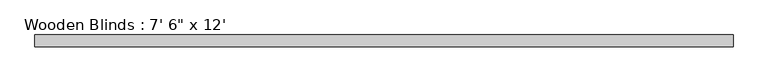
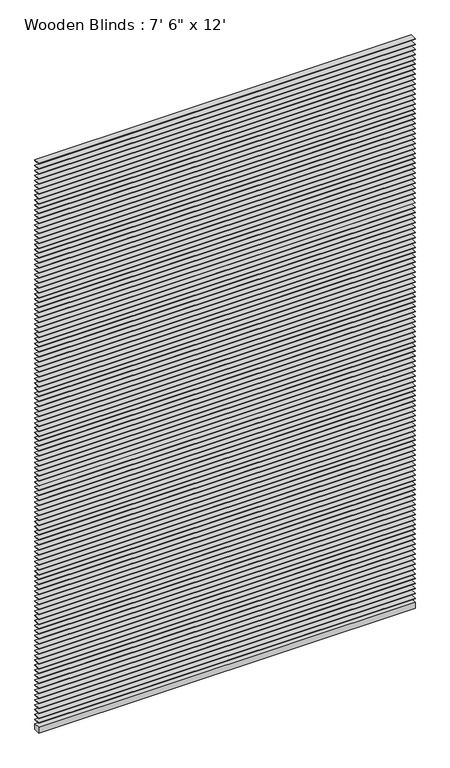
"""IFC4 building model written with IfcOpenShell, lengths in millimetres: furniture geometry."""

from ifc_helpers import new_model, si_unit, frame, origin, origin_with_axes, place, context, project, spatial, polyline, outline, extrude, source, transform, mapped, element, save


def furniture_480b9389(model_context):
    return source(origin(), model_context, "Body", "SweptSolid", [
        extrude(outline(polyline([(2286.0, 38.1), (2286.0, 0.0), (0.0, 0.0), (0.0, 38.1), (2286.0, 38.1)])), frame((0.0, 0.0, 3617.8790576), z_axis=(0.0, 0.0, 1.0), x_axis=(1.0, 0.0, 0.0)), (0.0, 0.0, 1.0), 3.175),
        extrude(outline(polyline([(2286.0, 38.1), (2286.0, 0.0), (0.0, 0.0), (0.0, 38.1), (2286.0, 38.1)])), frame((0.0, 0.0, 3586.1290576), z_axis=(0.0, 0.0, 1.0), x_axis=(1.0, 0.0, 0.0)), (0.0, 0.0, 1.0), 3.175),
        extrude(outline(polyline([(2286.0, 38.1), (2286.0, 0.0), (0.0, 0.0), (0.0, 38.1), (2286.0, 38.1)])), frame((0.0, 0.0, 3554.3790576), z_axis=(0.0, 0.0, 1.0), x_axis=(1.0, 0.0, 0.0)), (0.0, 0.0, 1.0), 3.175),
        extrude(outline(polyline([(2286.0, 38.1), (2286.0, 0.0), (0.0, 0.0), (0.0, 38.1), (2286.0, 38.1)])), frame((0.0, 0.0, 3522.6290576), z_axis=(0.0, 0.0, 1.0), x_axis=(1.0, 0.0, 0.0)), (0.0, 0.0, 1.0), 3.175),
        extrude(outline(polyline([(2286.0, 38.1), (2286.0, 0.0), (0.0, 0.0), (0.0, 38.1), (2286.0, 38.1)])), frame((0.0, 0.0, 3490.8790576), z_axis=(0.0, 0.0, 1.0), x_axis=(1.0, 0.0, 0.0)), (0.0, 0.0, 1.0), 3.175),
        extrude(outline(polyline([(2286.0, 38.1), (2286.0, 0.0), (0.0, 0.0), (0.0, 38.1), (2286.0, 38.1)])), frame((0.0, 0.0, 3459.1290576), z_axis=(0.0, 0.0, 1.0), x_axis=(1.0, 0.0, 0.0)), (0.0, 0.0, 1.0), 3.175),
        extrude(outline(polyline([(2286.0, 38.1), (2286.0, 0.0), (0.0, 0.0), (0.0, 38.1), (2286.0, 38.1)])), frame((0.0, 0.0, 3427.3790576), z_axis=(0.0, 0.0, 1.0), x_axis=(1.0, 0.0, 0.0)), (0.0, 0.0, 1.0), 3.175),
        extrude(outline(polyline([(2286.0, 38.1), (2286.0, 0.0), (0.0, 0.0), (0.0, 38.1), (2286.0, 38.1)])), frame((0.0, 0.0, 3395.6290576), z_axis=(0.0, 0.0, 1.0), x_axis=(1.0, 0.0, 0.0)), (0.0, 0.0, 1.0), 3.175),
        extrude(outline(polyline([(2286.0, 38.1), (2286.0, 0.0), (0.0, 0.0), (0.0, 38.1), (2286.0, 38.1)])), frame((0.0, 0.0, 3363.8790576), z_axis=(0.0, 0.0, 1.0), x_axis=(1.0, 0.0, 0.0)), (0.0, 0.0, 1.0), 3.175),
        extrude(outline(polyline([(2286.0, 38.1), (2286.0, 0.0), (0.0, 0.0), (0.0, 38.1), (2286.0, 38.1)])), frame((0.0, 0.0, 3332.1290576), z_axis=(0.0, 0.0, 1.0), x_axis=(1.0, 0.0, 0.0)), (0.0, 0.0, 1.0), 3.175),
        extrude(outline(polyline([(2286.0, 38.1), (2286.0, 0.0), (0.0, 0.0), (0.0, 38.1), (2286.0, 38.1)])), frame((0.0, 0.0, 3300.3790576), z_axis=(0.0, 0.0, 1.0), x_axis=(1.0, 0.0, 0.0)), (0.0, 0.0, 1.0), 3.175),
        extrude(outline(polyline([(2286.0, 38.1), (2286.0, 0.0), (0.0, 0.0), (0.0, 38.1), (2286.0, 38.1)])), frame((0.0, 0.0, 3268.6290576), z_axis=(0.0, 0.0, 1.0), x_axis=(1.0, 0.0, 0.0)), (0.0, 0.0, 1.0), 3.175),
        extrude(outline(polyline([(2286.0, 38.1), (2286.0, 0.0), (0.0, 0.0), (0.0, 38.1), (2286.0, 38.1)])), frame((0.0, 0.0, 3236.8790576), z_axis=(0.0, 0.0, 1.0), x_axis=(1.0, 0.0, 0.0)), (0.0, 0.0, 1.0), 3.175),
        extrude(outline(polyline([(2286.0, 38.1), (2286.0, 0.0), (0.0, 0.0), (0.0, 38.1), (2286.0, 38.1)])), frame((0.0, 0.0, 3205.1290576), z_axis=(0.0, 0.0, 1.0), x_axis=(1.0, 0.0, 0.0)), (0.0, 0.0, 1.0), 3.175),
        extrude(outline(polyline([(2286.0, 38.1), (2286.0, 0.0), (0.0, 0.0), (0.0, 38.1), (2286.0, 38.1)])), frame((0.0, 0.0, 3173.3790576), z_axis=(0.0, 0.0, 1.0), x_axis=(1.0, 0.0, 0.0)), (0.0, 0.0, 1.0), 3.175),
        extrude(outline(polyline([(2286.0, 38.1), (2286.0, 0.0), (0.0, 0.0), (0.0, 38.1), (2286.0, 38.1)])), frame((0.0, 0.0, 3141.6290576), z_axis=(0.0, 0.0, 1.0), x_axis=(1.0, 0.0, 0.0)), (0.0, 0.0, 1.0), 3.175),
        extrude(outline(polyline([(2286.0, 38.1), (2286.0, 0.0), (0.0, 0.0), (0.0, 38.1), (2286.0, 38.1)])), frame((0.0, 0.0, 3109.8790576), z_axis=(0.0, 0.0, 1.0), x_axis=(1.0, 0.0, 0.0)), (0.0, 0.0, 1.0), 3.175),
        extrude(outline(polyline([(2286.0, 38.1), (2286.0, 0.0), (0.0, 0.0), (0.0, 38.1), (2286.0, 38.1)])), frame((0.0, 0.0, 3078.1290576), z_axis=(0.0, 0.0, 1.0), x_axis=(1.0, 0.0, 0.0)), (0.0, 0.0, 1.0), 3.175),
        extrude(outline(polyline([(2286.0, 38.1), (2286.0, 0.0), (0.0, 0.0), (0.0, 38.1), (2286.0, 38.1)])), frame((0.0, 0.0, 3046.3790576), z_axis=(0.0, 0.0, 1.0), x_axis=(1.0, 0.0, 0.0)), (0.0, 0.0, 1.0), 3.175),
        extrude(outline(polyline([(2286.0, 38.1), (2286.0, 0.0), (0.0, 0.0), (0.0, 38.1), (2286.0, 38.1)])), frame((0.0, 0.0, 3014.6290576), z_axis=(0.0, 0.0, 1.0), x_axis=(1.0, 0.0, 0.0)), (0.0, 0.0, 1.0), 3.175),
        extrude(outline(polyline([(2286.0, 38.1), (2286.0, 0.0), (0.0, 0.0), (0.0, 38.1), (2286.0, 38.1)])), frame((0.0, 0.0, 2982.8790576), z_axis=(0.0, 0.0, 1.0), x_axis=(1.0, 0.0, 0.0)), (0.0, 0.0, 1.0), 3.175),
        extrude(outline(polyline([(2286.0, 38.1), (2286.0, 0.0), (0.0, 0.0), (0.0, 38.1), (2286.0, 38.1)])), frame((0.0, 0.0, 2951.1290576), z_axis=(0.0, 0.0, 1.0), x_axis=(1.0, 0.0, 0.0)), (0.0, 0.0, 1.0), 3.175),
        extrude(outline(polyline([(2286.0, 38.1), (2286.0, 0.0), (0.0, 0.0), (0.0, 38.1), (2286.0, 38.1)])), frame((0.0, 0.0, 2919.3790576), z_axis=(0.0, 0.0, 1.0), x_axis=(1.0, 0.0, 0.0)), (0.0, 0.0, 1.0), 3.175),
        extrude(outline(polyline([(2286.0, 38.1), (2286.0, 0.0), (0.0, 0.0), (0.0, 38.1), (2286.0, 38.1)])), frame((0.0, 0.0, 2887.6290576), z_axis=(0.0, 0.0, 1.0), x_axis=(1.0, 0.0, 0.0)), (0.0, 0.0, 1.0), 3.175),
        extrude(outline(polyline([(2286.0, 38.1), (2286.0, 0.0), (0.0, 0.0), (0.0, 38.1), (2286.0, 38.1)])), frame((0.0, 0.0, 2855.8790576), z_axis=(0.0, 0.0, 1.0), x_axis=(1.0, 0.0, 0.0)), (0.0, 0.0, 1.0), 3.175),
        extrude(outline(polyline([(2286.0, 38.1), (2286.0, 0.0), (0.0, 0.0), (0.0, 38.1), (2286.0, 38.1)])), frame((0.0, 0.0, 2824.1290576), z_axis=(0.0, 0.0, 1.0), x_axis=(1.0, 0.0, 0.0)), (0.0, 0.0, 1.0), 3.175),
        extrude(outline(polyline([(2286.0, 38.1), (2286.0, 0.0), (0.0, 0.0), (0.0, 38.1), (2286.0, 38.1)])), frame((0.0, 0.0, 2792.3790576), z_axis=(0.0, 0.0, 1.0), x_axis=(1.0, 0.0, 0.0)), (0.0, 0.0, 1.0), 3.175),
        extrude(outline(polyline([(2286.0, 38.1), (2286.0, 0.0), (0.0, 0.0), (0.0, 38.1), (2286.0, 38.1)])), frame((0.0, 0.0, 2760.6290576), z_axis=(0.0, 0.0, 1.0), x_axis=(1.0, 0.0, 0.0)), (0.0, 0.0, 1.0), 3.175),
        extrude(outline(polyline([(2286.0, 38.1), (2286.0, 0.0), (0.0, 0.0), (0.0, 38.1), (2286.0, 38.1)])), frame((0.0, 0.0, 2728.8790576), z_axis=(0.0, 0.0, 1.0), x_axis=(1.0, 0.0, 0.0)), (0.0, 0.0, 1.0), 3.175),
        extrude(outline(polyline([(2286.0, 38.1), (2286.0, 0.0), (0.0, 0.0), (0.0, 38.1), (2286.0, 38.1)])), frame((0.0, 0.0, 2697.1290576), z_axis=(0.0, 0.0, 1.0), x_axis=(1.0, 0.0, 0.0)), (0.0, 0.0, 1.0), 3.175),
        extrude(outline(polyline([(2286.0, 38.1), (2286.0, 0.0), (0.0, 0.0), (0.0, 38.1), (2286.0, 38.1)])), frame((0.0, 0.0, 2665.3790576), z_axis=(0.0, 0.0, 1.0), x_axis=(1.0, 0.0, 0.0)), (0.0, 0.0, 1.0), 3.175),
        extrude(outline(polyline([(2286.0, 38.1), (2286.0, 0.0), (0.0, 0.0), (0.0, 38.1), (2286.0, 38.1)])), frame((0.0, 0.0, 2633.6290576), z_axis=(0.0, 0.0, 1.0), x_axis=(1.0, 0.0, 0.0)), (0.0, 0.0, 1.0), 3.175),
        extrude(outline(polyline([(2286.0, 38.1), (2286.0, 0.0), (0.0, 0.0), (0.0, 38.1), (2286.0, 38.1)])), frame((0.0, 0.0, 2601.8790576), z_axis=(0.0, 0.0, 1.0), x_axis=(1.0, 0.0, 0.0)), (0.0, 0.0, 1.0), 3.175),
        extrude(outline(polyline([(2286.0, 38.1), (2286.0, 0.0), (0.0, 0.0), (0.0, 38.1), (2286.0, 38.1)])), frame((0.0, 0.0, 2570.1290576), z_axis=(0.0, 0.0, 1.0), x_axis=(1.0, 0.0, 0.0)), (0.0, 0.0, 1.0), 3.175),
        extrude(outline(polyline([(2286.0, 38.1), (2286.0, 0.0), (0.0, 0.0), (0.0, 38.1), (2286.0, 38.1)])), frame((0.0, 0.0, 2538.3790576), z_axis=(0.0, 0.0, 1.0), x_axis=(1.0, 0.0, 0.0)), (0.0, 0.0, 1.0), 3.175),
        extrude(outline(polyline([(2286.0, 38.1), (2286.0, 0.0), (0.0, 0.0), (0.0, 38.1), (2286.0, 38.1)])), frame((0.0, 0.0, 2506.6290576), z_axis=(0.0, 0.0, 1.0), x_axis=(1.0, 0.0, 0.0)), (0.0, 0.0, 1.0), 3.175),
        extrude(outline(polyline([(2286.0, 38.1), (2286.0, 0.0), (0.0, 0.0), (0.0, 38.1), (2286.0, 38.1)])), frame((0.0, 0.0, 2474.8790576), z_axis=(0.0, 0.0, 1.0), x_axis=(1.0, 0.0, 0.0)), (0.0, 0.0, 1.0), 3.175),
        extrude(outline(polyline([(2286.0, 38.1), (2286.0, 0.0), (0.0, 0.0), (0.0, 38.1), (2286.0, 38.1)])), frame((0.0, 0.0, 2443.1290576), z_axis=(0.0, 0.0, 1.0), x_axis=(1.0, 0.0, 0.0)), (0.0, 0.0, 1.0), 3.175),
        extrude(outline(polyline([(2286.0, 38.1), (2286.0, 0.0), (0.0, 0.0), (0.0, 38.1), (2286.0, 38.1)])), frame((0.0, 0.0, 2411.3790576), z_axis=(0.0, 0.0, 1.0), x_axis=(1.0, 0.0, 0.0)), (0.0, 0.0, 1.0), 3.175),
        extrude(outline(polyline([(2286.0, 38.1), (2286.0, 0.0), (0.0, 0.0), (0.0, 38.1), (2286.0, 38.1)])), frame((0.0, 0.0, 2379.6290576), z_axis=(0.0, 0.0, 1.0), x_axis=(1.0, 0.0, 0.0)), (0.0, 0.0, 1.0), 3.175),
        extrude(outline(polyline([(2286.0, 38.1), (2286.0, 0.0), (0.0, 0.0), (0.0, 38.1), (2286.0, 38.1)])), frame((0.0, 0.0, 2347.8790576), z_axis=(0.0, 0.0, 1.0), x_axis=(1.0, 0.0, 0.0)), (0.0, 0.0, 1.0), 3.175),
        extrude(outline(polyline([(2286.0, 38.1), (2286.0, 0.0), (0.0, 0.0), (0.0, 38.1), (2286.0, 38.1)])), frame((0.0, 0.0, 2316.1290576), z_axis=(0.0, 0.0, 1.0), x_axis=(1.0, 0.0, 0.0)), (0.0, 0.0, 1.0), 3.175),
        extrude(outline(polyline([(2286.0, 38.1), (2286.0, 0.0), (0.0, 0.0), (0.0, 38.1), (2286.0, 38.1)])), frame((0.0, 0.0, 2284.3790576), z_axis=(0.0, 0.0, 1.0), x_axis=(1.0, 0.0, 0.0)), (0.0, 0.0, 1.0), 3.175),
        extrude(outline(polyline([(2286.0, 38.1), (2286.0, 0.0), (0.0, 0.0), (0.0, 38.1), (2286.0, 38.1)])), frame((0.0, 0.0, 2252.6290576), z_axis=(0.0, 0.0, 1.0), x_axis=(1.0, 0.0, 0.0)), (0.0, 0.0, 1.0), 3.175),
        extrude(outline(polyline([(2286.0, 38.1), (2286.0, 0.0), (0.0, 0.0), (0.0, 38.1), (2286.0, 38.1)])), frame((0.0, 0.0, 2220.8790576), z_axis=(0.0, 0.0, 1.0), x_axis=(1.0, 0.0, 0.0)), (0.0, 0.0, 1.0), 3.175),
        extrude(outline(polyline([(2286.0, 38.1), (2286.0, 0.0), (0.0, 0.0), (0.0, 38.1), (2286.0, 38.1)])), frame((0.0, 0.0, 2189.1290576), z_axis=(0.0, 0.0, 1.0), x_axis=(1.0, 0.0, 0.0)), (0.0, 0.0, 1.0), 3.175),
        extrude(outline(polyline([(2286.0, 38.1), (2286.0, 0.0), (0.0, 0.0), (0.0, 38.1), (2286.0, 38.1)])), frame((0.0, 0.0, 2157.3790576), z_axis=(0.0, 0.0, 1.0), x_axis=(1.0, 0.0, 0.0)), (0.0, 0.0, 1.0), 3.175),
        extrude(outline(polyline([(2286.0, 38.1), (2286.0, 0.0), (0.0, 0.0), (0.0, 38.1), (2286.0, 38.1)])), frame((0.0, 0.0, 2125.6290576), z_axis=(0.0, 0.0, 1.0), x_axis=(1.0, 0.0, 0.0)), (0.0, 0.0, 1.0), 3.175),
        extrude(outline(polyline([(2286.0, 38.1), (2286.0, 0.0), (0.0, 0.0), (0.0, 38.1), (2286.0, 38.1)])), frame((0.0, 0.0, 2093.8790576), z_axis=(0.0, 0.0, 1.0), x_axis=(1.0, 0.0, 0.0)), (0.0, 0.0, 1.0), 3.175),
        extrude(outline(polyline([(2286.0, 38.1), (2286.0, 0.0), (0.0, 0.0), (0.0, 38.1), (2286.0, 38.1)])), frame((0.0, 0.0, 2062.1290576), z_axis=(0.0, 0.0, 1.0), x_axis=(1.0, 0.0, 0.0)), (0.0, 0.0, 1.0), 3.175),
        extrude(outline(polyline([(2286.0, 38.1), (2286.0, 0.0), (0.0, 0.0), (0.0, 38.1), (2286.0, 38.1)])), frame((0.0, 0.0, 2030.3790576), z_axis=(0.0, 0.0, 1.0), x_axis=(1.0, 0.0, 0.0)), (0.0, 0.0, 1.0), 3.175),
        extrude(outline(polyline([(2286.0, 38.1), (2286.0, 0.0), (0.0, 0.0), (0.0, 38.1), (2286.0, 38.1)])), frame((0.0, 0.0, 1998.6290576), z_axis=(0.0, 0.0, 1.0), x_axis=(1.0, 0.0, 0.0)), (0.0, 0.0, 1.0), 3.175),
        extrude(outline(polyline([(2286.0, 38.1), (2286.0, 0.0), (0.0, 0.0), (0.0, 38.1), (2286.0, 38.1)])), frame((0.0, 0.0, 1966.8790576), z_axis=(0.0, 0.0, 1.0), x_axis=(1.0, 0.0, 0.0)), (0.0, 0.0, 1.0), 3.175),
        extrude(outline(polyline([(2286.0, 38.1), (2286.0, 0.0), (0.0, 0.0), (0.0, 38.1), (2286.0, 38.1)])), frame((0.0, 0.0, 1935.1290576), z_axis=(0.0, 0.0, 1.0), x_axis=(1.0, 0.0, 0.0)), (0.0, 0.0, 1.0), 3.175),
        extrude(outline(polyline([(2286.0, 38.1), (2286.0, 0.0), (0.0, 0.0), (0.0, 38.1), (2286.0, 38.1)])), frame((0.0, 0.0, 1903.3790576), z_axis=(0.0, 0.0, 1.0), x_axis=(1.0, 0.0, 0.0)), (0.0, 0.0, 1.0), 3.175),
        extrude(outline(polyline([(2286.0, 38.1), (2286.0, 0.0), (0.0, 0.0), (0.0, 38.1), (2286.0, 38.1)])), frame((0.0, 0.0, 1871.6290576), z_axis=(0.0, 0.0, 1.0), x_axis=(1.0, 0.0, 0.0)), (0.0, 0.0, 1.0), 3.175),
        extrude(outline(polyline([(2286.0, 38.1), (2286.0, 0.0), (0.0, 0.0), (0.0, 38.1), (2286.0, 38.1)])), frame((0.0, 0.0, 1839.8790576), z_axis=(0.0, 0.0, 1.0), x_axis=(1.0, 0.0, 0.0)), (0.0, 0.0, 1.0), 3.175),
        extrude(outline(polyline([(2286.0, 38.1), (2286.0, 0.0), (0.0, 0.0), (0.0, 38.1), (2286.0, 38.1)])), frame((0.0, 0.0, 1808.1290576), z_axis=(0.0, 0.0, 1.0), x_axis=(1.0, 0.0, 0.0)), (0.0, 0.0, 1.0), 3.175),
        extrude(outline(polyline([(2286.0, 38.1), (2286.0, 0.0), (0.0, 0.0), (0.0, 38.1), (2286.0, 38.1)])), frame((0.0, 0.0, 1776.3790576), z_axis=(0.0, 0.0, 1.0), x_axis=(1.0, 0.0, 0.0)), (0.0, 0.0, 1.0), 3.175),
        extrude(outline(polyline([(2286.0, 38.1), (2286.0, 0.0), (0.0, 0.0), (0.0, 38.1), (2286.0, 38.1)])), frame((0.0, 0.0, 1744.6290576), z_axis=(0.0, 0.0, 1.0), x_axis=(1.0, 0.0, 0.0)), (0.0, 0.0, 1.0), 3.175),
        extrude(outline(polyline([(2286.0, 38.1), (2286.0, 0.0), (0.0, 0.0), (0.0, 38.1), (2286.0, 38.1)])), frame((0.0, 0.0, 1712.8790576), z_axis=(0.0, 0.0, 1.0), x_axis=(1.0, 0.0, 0.0)), (0.0, 0.0, 1.0), 3.175),
        extrude(outline(polyline([(2286.0, 38.1), (2286.0, 0.0), (0.0, 0.0), (0.0, 38.1), (2286.0, 38.1)])), frame((0.0, 0.0, 1681.1290576), z_axis=(0.0, 0.0, 1.0), x_axis=(1.0, 0.0, 0.0)), (0.0, 0.0, 1.0), 3.175),
        extrude(outline(polyline([(2286.0, 38.1), (2286.0, 0.0), (0.0, 0.0), (0.0, 38.1), (2286.0, 38.1)])), frame((0.0, 0.0, 1649.3790576), z_axis=(0.0, 0.0, 1.0), x_axis=(1.0, 0.0, 0.0)), (0.0, 0.0, 1.0), 3.175),
        extrude(outline(polyline([(2286.0, 38.1), (2286.0, 0.0), (0.0, 0.0), (0.0, 38.1), (2286.0, 38.1)])), frame((0.0, 0.0, 1617.6290576), z_axis=(0.0, 0.0, 1.0), x_axis=(1.0, 0.0, 0.0)), (0.0, 0.0, 1.0), 3.175),
        extrude(outline(polyline([(2286.0, 38.1), (2286.0, 0.0), (0.0, 0.0), (0.0, 38.1), (2286.0, 38.1)])), frame((0.0, 0.0, 1585.8790576), z_axis=(0.0, 0.0, 1.0), x_axis=(1.0, 0.0, 0.0)), (0.0, 0.0, 1.0), 3.175),
        extrude(outline(polyline([(2286.0, 38.1), (2286.0, 0.0), (0.0, 0.0), (0.0, 38.1), (2286.0, 38.1)])), frame((0.0, 0.0, 1554.1290576), z_axis=(0.0, 0.0, 1.0), x_axis=(1.0, 0.0, 0.0)), (0.0, 0.0, 1.0), 3.175),
        extrude(outline(polyline([(2286.0, 38.1), (2286.0, 0.0), (0.0, 0.0), (0.0, 38.1), (2286.0, 38.1)])), frame((0.0, 0.0, 1522.3790576), z_axis=(0.0, 0.0, 1.0), x_axis=(1.0, 0.0, 0.0)), (0.0, 0.0, 1.0), 3.175),
        extrude(outline(polyline([(2286.0, 38.1), (2286.0, 0.0), (0.0, 0.0), (0.0, 38.1), (2286.0, 38.1)])), frame((0.0, 0.0, 1490.6290576), z_axis=(0.0, 0.0, 1.0), x_axis=(1.0, 0.0, 0.0)), (0.0, 0.0, 1.0), 3.175),
        extrude(outline(polyline([(2286.0, 38.1), (2286.0, 0.0), (0.0, 0.0), (0.0, 38.1), (2286.0, 38.1)])), frame((0.0, 0.0, 1458.8790576), z_axis=(0.0, 0.0, 1.0), x_axis=(1.0, 0.0, 0.0)), (0.0, 0.0, 1.0), 3.175),
        extrude(outline(polyline([(2286.0, 38.1), (2286.0, 0.0), (0.0, 0.0), (0.0, 38.1), (2286.0, 38.1)])), frame((0.0, 0.0, 1427.1290576), z_axis=(0.0, 0.0, 1.0), x_axis=(1.0, 0.0, 0.0)), (0.0, 0.0, 1.0), 3.175),
        extrude(outline(polyline([(2286.0, 38.1), (2286.0, 0.0), (0.0, 0.0), (0.0, 38.1), (2286.0, 38.1)])), frame((0.0, 0.0, 1395.3790576), z_axis=(0.0, 0.0, 1.0), x_axis=(1.0, 0.0, 0.0)), (0.0, 0.0, 1.0), 3.175),
        extrude(outline(polyline([(2286.0, 38.1), (2286.0, 0.0), (0.0, 0.0), (0.0, 38.1), (2286.0, 38.1)])), frame((0.0, 0.0, 1363.6290576), z_axis=(0.0, 0.0, 1.0), x_axis=(1.0, 0.0, 0.0)), (0.0, 0.0, 1.0), 3.175),
        extrude(outline(polyline([(2286.0, 38.1), (2286.0, 0.0), (0.0, 0.0), (0.0, 38.1), (2286.0, 38.1)])), frame((0.0, 0.0, 1331.8790576), z_axis=(0.0, 0.0, 1.0), x_axis=(1.0, 0.0, 0.0)), (0.0, 0.0, 1.0), 3.175),
        extrude(outline(polyline([(2286.0, 38.1), (2286.0, 0.0), (0.0, 0.0), (0.0, 38.1), (2286.0, 38.1)])), frame((0.0, 0.0, 1300.1290576), z_axis=(0.0, 0.0, 1.0), x_axis=(1.0, 0.0, 0.0)), (0.0, 0.0, 1.0), 3.175),
        extrude(outline(polyline([(2286.0, 38.1), (2286.0, 0.0), (0.0, 0.0), (0.0, 38.1), (2286.0, 38.1)])), frame((0.0, 0.0, 1268.3790576), z_axis=(0.0, 0.0, 1.0), x_axis=(1.0, 0.0, 0.0)), (0.0, 0.0, 1.0), 3.175),
        extrude(outline(polyline([(2286.0, 38.1), (2286.0, 0.0), (0.0, 0.0), (0.0, 38.1), (2286.0, 38.1)])), frame((0.0, 0.0, 1236.6290576), z_axis=(0.0, 0.0, 1.0), x_axis=(1.0, 0.0, 0.0)), (0.0, 0.0, 1.0), 3.175),
        extrude(outline(polyline([(2286.0, 38.1), (2286.0, 0.0), (0.0, 0.0), (0.0, 38.1), (2286.0, 38.1)])), frame((0.0, 0.0, 1204.8790576), z_axis=(0.0, 0.0, 1.0), x_axis=(1.0, 0.0, 0.0)), (0.0, 0.0, 1.0), 3.175),
        extrude(outline(polyline([(2286.0, 38.1), (2286.0, 0.0), (0.0, 0.0), (0.0, 38.1), (2286.0, 38.1)])), frame((0.0, 0.0, 1173.1290576), z_axis=(0.0, 0.0, 1.0), x_axis=(1.0, 0.0, 0.0)), (0.0, 0.0, 1.0), 3.175),
        extrude(outline(polyline([(2286.0, 38.1), (2286.0, 0.0), (0.0, 0.0), (0.0, 38.1), (2286.0, 38.1)])), frame((0.0, 0.0, 1141.3790576), z_axis=(0.0, 0.0, 1.0), x_axis=(1.0, 0.0, 0.0)), (0.0, 0.0, 1.0), 3.175),
        extrude(outline(polyline([(2286.0, 38.1), (2286.0, 0.0), (0.0, 0.0), (0.0, 38.1), (2286.0, 38.1)])), frame((0.0, 0.0, 1109.6290576), z_axis=(0.0, 0.0, 1.0), x_axis=(1.0, 0.0, 0.0)), (0.0, 0.0, 1.0), 3.175),
        extrude(outline(polyline([(2286.0, 38.1), (2286.0, 0.0), (0.0, 0.0), (0.0, 38.1), (2286.0, 38.1)])), frame((0.0, 0.0, 1077.8790576), z_axis=(0.0, 0.0, 1.0), x_axis=(1.0, 0.0, 0.0)), (0.0, 0.0, 1.0), 3.175),
        extrude(outline(polyline([(2286.0, 38.1), (2286.0, 0.0), (0.0, 0.0), (0.0, 38.1), (2286.0, 38.1)])), frame((0.0, 0.0, 1046.1290576), z_axis=(0.0, 0.0, 1.0), x_axis=(1.0, 0.0, 0.0)), (0.0, 0.0, 1.0), 3.175),
        extrude(outline(polyline([(2286.0, 38.1), (2286.0, 0.0), (0.0, 0.0), (0.0, 38.1), (2286.0, 38.1)])), frame((0.0, 0.0, 1014.3790576), z_axis=(0.0, 0.0, 1.0), x_axis=(1.0, 0.0, 0.0)), (0.0, 0.0, 1.0), 3.175),
        extrude(outline(polyline([(2286.0, 38.1), (2286.0, 0.0), (0.0, 0.0), (0.0, 38.1), (2286.0, 38.1)])), frame((0.0, 0.0, 982.6290576), z_axis=(0.0, 0.0, 1.0), x_axis=(1.0, 0.0, 0.0)), (0.0, 0.0, 1.0), 3.175),
        extrude(outline(polyline([(2286.0, 38.1), (2286.0, 0.0), (0.0, 0.0), (0.0, 38.1), (2286.0, 38.1)])), frame((0.0, 0.0, 950.8790576), z_axis=(0.0, 0.0, 1.0), x_axis=(1.0, 0.0, 0.0)), (0.0, 0.0, 1.0), 3.175),
        extrude(outline(polyline([(2286.0, 38.1), (2286.0, 0.0), (0.0, 0.0), (0.0, 38.1), (2286.0, 38.1)])), frame((0.0, 0.0, 919.1290576), z_axis=(0.0, 0.0, 1.0), x_axis=(1.0, 0.0, 0.0)), (0.0, 0.0, 1.0), 3.175),
        extrude(outline(polyline([(2286.0, 38.1), (2286.0, 0.0), (0.0, 0.0), (0.0, 38.1), (2286.0, 38.1)])), frame((0.0, 0.0, 887.3790576), z_axis=(0.0, 0.0, 1.0), x_axis=(1.0, 0.0, 0.0)), (0.0, 0.0, 1.0), 3.175),
        extrude(outline(polyline([(2286.0, 38.1), (2286.0, 0.0), (0.0, 0.0), (0.0, 38.1), (2286.0, 38.1)])), frame((0.0, 0.0, 855.6290576), z_axis=(0.0, 0.0, 1.0), x_axis=(1.0, 0.0, 0.0)), (0.0, 0.0, 1.0), 3.175),
        extrude(outline(polyline([(2286.0, 38.1), (2286.0, 0.0), (0.0, 0.0), (0.0, 38.1), (2286.0, 38.1)])), frame((0.0, 0.0, 823.8790576), z_axis=(0.0, 0.0, 1.0), x_axis=(1.0, 0.0, 0.0)), (0.0, 0.0, 1.0), 3.175),
        extrude(outline(polyline([(2286.0, 38.1), (2286.0, 0.0), (0.0, 0.0), (0.0, 38.1), (2286.0, 38.1)])), frame((0.0, 0.0, 792.1290576), z_axis=(0.0, 0.0, 1.0), x_axis=(1.0, 0.0, 0.0)), (0.0, 0.0, 1.0), 3.175),
        extrude(outline(polyline([(2286.0, 38.1), (2286.0, 0.0), (0.0, 0.0), (0.0, 38.1), (2286.0, 38.1)])), frame((0.0, 0.0, 760.3790576), z_axis=(0.0, 0.0, 1.0), x_axis=(1.0, 0.0, 0.0)), (0.0, 0.0, 1.0), 3.175),
        extrude(outline(polyline([(2286.0, 38.1), (2286.0, 0.0), (0.0, 0.0), (0.0, 38.1), (2286.0, 38.1)])), frame((0.0, 0.0, 728.6290576), z_axis=(0.0, 0.0, 1.0), x_axis=(1.0, 0.0, 0.0)), (0.0, 0.0, 1.0), 3.175),
        extrude(outline(polyline([(2286.0, 38.1), (2286.0, 0.0), (0.0, 0.0), (0.0, 38.1), (2286.0, 38.1)])), frame((0.0, 0.0, 696.8790576), z_axis=(0.0, 0.0, 1.0), x_axis=(1.0, 0.0, 0.0)), (0.0, 0.0, 1.0), 3.175),
        extrude(outline(polyline([(2286.0, 38.1), (2286.0, 0.0), (0.0, 0.0), (0.0, 38.1), (2286.0, 38.1)])), frame((0.0, 0.0, 665.1290576), z_axis=(0.0, 0.0, 1.0), x_axis=(1.0, 0.0, 0.0)), (0.0, 0.0, 1.0), 3.175),
        extrude(outline(polyline([(2286.0, 38.1), (2286.0, 0.0), (0.0, 0.0), (0.0, 38.1), (2286.0, 38.1)])), frame((0.0, 0.0, 633.3790576), z_axis=(0.0, 0.0, 1.0), x_axis=(1.0, 0.0, 0.0)), (0.0, 0.0, 1.0), 3.175),
        extrude(outline(polyline([(2286.0, 38.1), (2286.0, 0.0), (0.0, 0.0), (0.0, 38.1), (2286.0, 38.1)])), frame((0.0, 0.0, 601.6290576), z_axis=(0.0, 0.0, 1.0), x_axis=(1.0, 0.0, 0.0)), (0.0, 0.0, 1.0), 3.175),
        extrude(outline(polyline([(2286.0, 38.1), (2286.0, 0.0), (0.0, 0.0), (0.0, 38.1), (2286.0, 38.1)])), frame((0.0, 0.0, 569.8790576), z_axis=(0.0, 0.0, 1.0), x_axis=(1.0, 0.0, 0.0)), (0.0, 0.0, 1.0), 3.175),
        extrude(outline(polyline([(2286.0, 38.1), (2286.0, 0.0), (0.0, 0.0), (0.0, 38.1), (2286.0, 38.1)])), frame((0.0, 0.0, 538.1290576), z_axis=(0.0, 0.0, 1.0), x_axis=(1.0, 0.0, 0.0)), (0.0, 0.0, 1.0), 3.175),
        extrude(outline(polyline([(2286.0, 38.1), (2286.0, 0.0), (0.0, 0.0), (0.0, 38.1), (2286.0, 38.1)])), frame((0.0, 0.0, 506.3790576), z_axis=(0.0, 0.0, 1.0), x_axis=(1.0, 0.0, 0.0)), (0.0, 0.0, 1.0), 3.175),
        extrude(outline(polyline([(2286.0, 38.1), (2286.0, 0.0), (0.0, 0.0), (0.0, 38.1), (2286.0, 38.1)])), frame((0.0, 0.0, 474.6290576), z_axis=(0.0, 0.0, 1.0), x_axis=(1.0, 0.0, 0.0)), (0.0, 0.0, 1.0), 3.175),
        extrude(outline(polyline([(2286.0, 38.1), (2286.0, 0.0), (0.0, 0.0), (0.0, 38.1), (2286.0, 38.1)])), frame((0.0, 0.0, 442.8790576), z_axis=(0.0, 0.0, 1.0), x_axis=(1.0, 0.0, 0.0)), (0.0, 0.0, 1.0), 3.175),
        extrude(outline(polyline([(2286.0, 38.1), (2286.0, 0.0), (0.0, 0.0), (0.0, 38.1), (2286.0, 38.1)])), frame((0.0, 0.0, 411.1290576), z_axis=(0.0, 0.0, 1.0), x_axis=(1.0, 0.0, 0.0)), (0.0, 0.0, 1.0), 3.175),
        extrude(outline(polyline([(2286.0, 38.1), (2286.0, 0.0), (0.0, 0.0), (0.0, 38.1), (2286.0, 38.1)])), frame((0.0, 0.0, 379.3790576), z_axis=(0.0, 0.0, 1.0), x_axis=(1.0, 0.0, 0.0)), (0.0, 0.0, 1.0), 3.175),
        extrude(outline(polyline([(2286.0, 38.1), (2286.0, 0.0), (0.0, 0.0), (0.0, 38.1), (2286.0, 38.1)])), frame((0.0, 0.0, 347.6290576), z_axis=(0.0, 0.0, 1.0), x_axis=(1.0, 0.0, 0.0)), (0.0, 0.0, 1.0), 3.175),
        extrude(outline(polyline([(2286.0, 38.1), (2286.0, 0.0), (0.0, 0.0), (0.0, 38.1), (2286.0, 38.1)])), frame((0.0, 0.0, 315.8790576), z_axis=(0.0, 0.0, 1.0), x_axis=(1.0, 0.0, 0.0)), (0.0, 0.0, 1.0), 3.175),
        extrude(outline(polyline([(2286.0, 38.1), (2286.0, 0.0), (0.0, 0.0), (0.0, 38.1), (2286.0, 38.1)])), frame((0.0, 0.0, 284.1290576), z_axis=(0.0, 0.0, 1.0), x_axis=(1.0, 0.0, 0.0)), (0.0, 0.0, 1.0), 3.175),
        extrude(outline(polyline([(2286.0, 38.1), (2286.0, 0.0), (0.0, 0.0), (0.0, 38.1), (2286.0, 38.1)])), frame((0.0, 0.0, 252.3790576), z_axis=(0.0, 0.0, 1.0), x_axis=(1.0, 0.0, 0.0)), (0.0, 0.0, 1.0), 3.175),
        extrude(outline(polyline([(2286.0, 38.1), (2286.0, 0.0), (0.0, 0.0), (0.0, 38.1), (2286.0, 38.1)])), frame((0.0, 0.0, 220.6290576), z_axis=(0.0, 0.0, 1.0), x_axis=(1.0, 0.0, 0.0)), (0.0, 0.0, 1.0), 3.175),
        extrude(outline(polyline([(2286.0, 38.1), (2286.0, 0.0), (0.0, 0.0), (0.0, 38.1), (2286.0, 38.1)])), frame((0.0, 0.0, 188.8790576), z_axis=(0.0, 0.0, 1.0), x_axis=(1.0, 0.0, 0.0)), (0.0, 0.0, 1.0), 3.175),
        extrude(outline(polyline([(2286.0, 38.1), (2286.0, 0.0), (0.0, 0.0), (0.0, 38.1), (2286.0, 38.1)])), frame((0.0, 0.0, 157.1290576), z_axis=(0.0, 0.0, 1.0), x_axis=(1.0, 0.0, 0.0)), (0.0, 0.0, 1.0), 3.175),
        extrude(outline(polyline([(2286.0, 38.1), (2286.0, 0.0), (0.0, 0.0), (0.0, 38.1), (2286.0, 38.1)])), frame((0.0, 0.0, 125.3790576), z_axis=(0.0, 0.0, 1.0), x_axis=(1.0, 0.0, 0.0)), (0.0, 0.0, 1.0), 3.175),
        extrude(outline(polyline([(2286.0, 38.1), (2286.0, 0.0), (0.0, 0.0), (0.0, 38.1), (2286.0, 38.1)])), frame((0.0, 0.0, 93.6290576), z_axis=(0.0, 0.0, 1.0), x_axis=(1.0, 0.0, 0.0)), (0.0, 0.0, 1.0), 3.175),
        extrude(outline(polyline([(2286.0, 38.1), (2286.0, 0.0), (0.0, 0.0), (0.0, 38.1), (2286.0, 38.1)])), frame((0.0, 0.0, 61.8790576), z_axis=(0.0, 0.0, 1.0), x_axis=(1.0, 0.0, 0.0)), (0.0, 0.0, 1.0), 3.175),
        extrude(outline(polyline([(2286.0, 38.1), (2286.0, 0.0), (0.0, 0.0), (0.0, 38.1), (2286.0, 38.1)])), frame((0.0, 0.0, 3651.25), z_axis=(0.0, 0.0, 1.0), x_axis=(1.0, 0.0, 0.0)), (0.0, 0.0, 1.0), 6.35),
        extrude(outline(polyline([(2286.0, 38.1), (2286.0, 0.0), (0.0, 0.0), (0.0, 38.1), (2286.0, 38.1)])), origin_with_axes(), (0.0, 0.0, 1.0), 38.1),
    ])


if __name__ == "__main__":
    model = new_model("IFC4")
    model_context = context("Model", 3, world=origin())
    ifc_project = project(units=[si_unit("LENGTHUNIT", "METRE", prefix="MILLI")], contexts=[model_context])
    site = spatial("IfcSite", under=ifc_project)
    building = spatial("IfcBuilding", under=site)
    placement = place(None, origin())
    furniture_shape = furniture_480b9389(model_context)
    element("IfcFurniture", 1, ObjectType="Wooden Blinds : 7' 6\" x 12'", at=placement, inside=building, context=model_context, shape_type="MappedRepresentation", body=[
        mapped(furniture_shape, transform((0.0, 0.0, 0.0), x_axis=(1.0, 0.0, 0.0), y_axis=(0.0, 1.0, 0.0), z_axis=(0.0, 0.0, 1.0))),
    ])
    save(model, "model.ifc")

# Revit data of these elements
# Type "Wooden Blinds : 7' 6\" x 12'"
#   Width = 7' - 6"
#   Slat Thickness = 0' - 0 1/8"
#   Height = 12' - 0"
#   Depth = 0' - 1 1/2"
#   Default Elevation = 4' - 0"
#   Blind Rotation = 90.00°
#   Number of Slats = 113
#   Slat = Metal - Chrome
#   Frame = Metal - Chrome
#   Assembly Code = ""
# Element 1 (IfcFurniture, "Wooden Blinds : 7' 6\" x 12'")
#   Materials on its faces: "Metal - Chrome"
# Materials
#   "Metal - Chrome": class "Metal", colour RGB 244 244 244, transparency 0, Comments = "Rendering appearance not upgraded Rendering appearance not upgraded ", Description = "Chrome"
